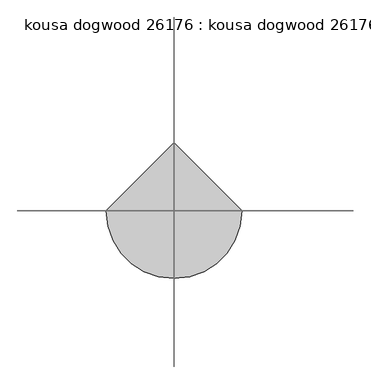
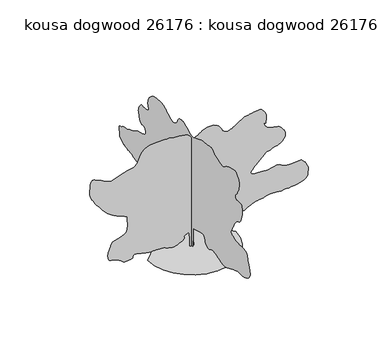
"""IFC4 building model written with IfcOpenShell, lengths in millimetres: proxy geometry, kousa dogwood 26176 : kousa dogwood 26176."""

from ifc_helpers import new_model, si_unit, origin, place, context, project, spatial, triangles, source, transform, mapped, element, save


def kousa_dogwood_26176_kousa_dogwood_26176_6f0fc0eb(model_context):
    return source(origin(), model_context, "Body", "Tessellation", [
        triangles([(0.0326291, 49.3377043, 0.0034665), (0.0326291, -50.8601768, 0.0034665), (0.0326291, -57.1220357, 331.9092828), (0.0326291, -57.1220357, 475.9424606), (0.0326291, -182.3693916, 513.516657), (0.0326291, -389.0262543, 582.4014421), (0.0326291, -489.2241354, 594.9261864), (0.0326291, -501.2738723, 584.1362563), (0.0326291, -513.1610827, 573.0186936), (0.0326291, -524.7180808, 561.2407062), (0.0326291, -535.7823037, 548.4797482), (0.0326291, -546.1886816, 534.4031001), (0.0326291, -555.7746517, 518.6830204), (0.0326291, -564.3725281, 500.9919491), (0.0326291, -570.4532979, 482.6074244), (0.0326291, -573.902615, 465.0966837), (0.0326291, -576.6965941, 448.573964), (0.0326291, -580.8037926, 433.1460176), (0.0326291, -588.2002524, 418.9245747), (0.0326291, -600.8519875, 406.0163146), (0.0326291, -620.7350761, 394.5304241), (0.0326291, -644.1412056, 383.9411722), (0.0326291, -666.1223494, 374.2282113), (0.0326291, -686.7903465, 366.2678687), (0.0326291, -706.251804, 360.9389425), (0.0326291, -724.6185608, 359.1126732), (0.0326291, -742.0023108, 361.6679315), (0.0326291, -758.5046465, 369.4834791), (0.0326291, -775.1569004, 379.6689039), (0.0326291, -792.794632, 388.8713219), (0.0326291, -811.2528076, 397.2532957), (0.0326291, -830.3688646, 404.9748811), (0.0326291, -849.9750807, 412.2062711), (0.0326291, -869.9141253, 419.1074487), (0.0326291, -890.0156599, 425.8435201), (0.0326291, -1008.9993856, 407.0551683), (0.0326291, -1041.2065767, 396.3388893), (0.0326291, -1073.4136951, 385.7318696), (0.0326291, -1105.6183428, 375.3432595), (0.0326291, -1137.8255339, 365.2823184), (0.0326291, -1170.032725, 355.6608127), (0.0326291, -1202.2373726, 346.587929), (0.0326291, -1234.4445637, 338.1703832), (0.0326291, -1267.7464554, 329.9534792), (0.0326291, -1303.0194477, 322.2852336), (0.0326291, -1339.935799, 316.4813364), (0.0326291, -1378.1679131, 313.8524271), (0.0326291, -1417.3854321, 315.7142684), (0.0326291, -1457.2609051, 323.382514), (0.0326291, -1497.4639744, 338.1703832), (0.0326291, -1798.0576904, 463.4177527), (0.0326291, -1820.2750843, 473.4227743), (0.0326291, -1840.0844856, 482.1121422), (0.0326291, -1859.675441, 489.7092802), (0.0326291, -1881.2374969, 496.4275475), (0.0326291, -1906.9626709, 502.488006), (0.0326291, -1939.0428349, 508.1115726), (0.0326291, -1979.6650646, 513.516657), (0.0326291, -2025.1640316, 517.2225354), (0.0326291, -2069.8934235, 518.6271372), (0.0326291, -2113.0912228, 519.2672144), (0.0326291, -2153.987709, 520.6743959), (0.0326291, -2191.8183941, 524.3802381), (0.0326291, -2225.8138481, 531.9189494), (0.0326291, -2255.2066761, 544.8272458), (0.0326291, -2282.9789635, 559.6176584), (0.0326291, -2311.7343304, 572.6529456), (0.0326291, -2340.1594849, 585.2513409), (0.0326291, -2366.9437511, 598.7234837), (0.0326291, -2390.7715118, 614.3901873), (0.0326291, -2410.3243881, 633.559584), (0.0326291, -2424.2918495, 657.5498348), (0.0326291, -2435.5745911, 680.3717703), (0.0326291, -2447.0782494, 697.4989952), (0.0326291, -2457.4845909, 712.4315866), (0.0326291, -2465.4806145, 728.6825569), (0.0326291, -2469.7527374, 749.7518377), (0.0326291, -2468.9856331, 779.1472092), (0.0326291, -2461.8660095, 820.3714371), (0.0326291, -2451.1117241, 863.1297283), (0.0326291, -2440.248143, 897.1276531), (0.0326291, -2429.166116, 925.8652159), (0.0326291, -2417.7564926, 952.8475805), (0.0326291, -2405.9073612, 981.5851433), (0.0326291, -2393.5095715, 1015.5830681), (0.0326291, -2380.4565891, 1058.3413593), (0.0326291, -2369.079958, 1104.2416826), (0.0326291, -2359.2400063, 1144.8817165), (0.0326291, -2347.0987415, 1179.6085213), (0.0326291, -2328.8234035, 1207.76189), (0.0326291, -2300.578616, 1228.6838688), (0.0326291, -2258.5314732, 1241.7191196), (0.0326291, -2198.8465988, 1246.21245), (0.0326291, -2132.0421009, 1246.3038689), (0.0326291, -2070.825634, 1246.94133), (0.0326291, -2014.6459236, 1248.6762531), (0.0326291, -1962.9595436, 1252.05439), (0.0326291, -1915.2150742, 1257.6220734), (0.0326291, -1870.8667637, 1265.9304325), (0.0326291, -1829.3682793, 1277.5230389), (0.0326291, -1789.1296017, 1289.3542934), (0.0326291, -1750.5318123, 1299.3237431), (0.0326291, -1715.9876999, 1309.4000175), (0.0326291, -1687.9080185, 1321.5614845), (0.0326291, -1668.7006153, 1337.7743031), (0.0326291, -1660.7782791, 1360.0120445), (0.0326291, -1666.546677, 1390.2455189), (0.0326291, -1677.3009624, 1417.6496601), (0.0326291, -1684.3291672, 1433.8802101), (0.0326291, -1690.0442253, 1444.6346409), (0.0326291, -1696.8539841, 1455.6073723), (0.0326291, -1707.1689068, 1472.4958763), (0.0326291, -1723.4020729, 1500.9971889), (0.0326291, -1747.9587135, 1546.8060207), (0.0326291, -1772.6957211, 1595.4241287), (0.0326291, -1790.2065708, 1631.3371983), (0.0326291, -1803.9910492, 1658.7057312), (0.0326291, -1817.5547562, 1681.6927002), (0.0326291, -1834.4076519, 1704.4587524), (0.0326291, -1858.0499588, 1731.1693314), (0.0326291, -1891.9919277, 1765.9877003), (0.0326291, -1930.3865318, 1797.7731148), (0.0326291, -1965.2784428, 1817.0720821), (0.0326291, -1996.9903152, 1830.5645725), (0.0326291, -2025.8549778, 1844.9333176), (0.0326291, -2052.2023521, 1866.8611942), (0.0326291, -2076.3577091, 1903.0281727), (0.0326291, -2098.6487904, 1960.119746), (0.0326291, -2116.6878056, 2031.8721977), (0.0326291, -2127.9349388, 2104.7193501), (0.0326291, -2132.4993404, 2174.3915508), (0.0326291, -2130.4901608, 2236.6139156), (0.0326291, -2122.0193115, 2287.1141762), (0.0326291, -2107.193327, 2321.6200642), (0.0326291, -2086.1239735, 2335.8617821), (0.0326291, -2061.2395912, 2337.8150059), (0.0326291, -2035.0395916, 2338.4550831), (0.0326291, -2007.744746, 2337.9979889), (0.0326291, -1979.5736458, 2336.6644947), (0.0326291, -1950.7445915, 2334.6756626), (0.0326291, -1921.4787907, 2332.2473225), (0.0326291, -1891.9919277, 2329.5982109), (0.0326291, -1876.0712425, 2337.7591953), (0.0326291, -1861.2452579, 2346.5781338), (0.0326291, -1848.6112907, 2356.7126896), (0.0326291, -1839.2640415, 2368.8157299), (0.0326291, -1834.2983562, 2383.5502956), (0.0326291, -1834.8089355, 2401.5691086), (0.0326291, -1841.8929508, 2423.534919), (0.0326291, -1852.3552483, 2443.6188675), (0.0326291, -1862.7057793, 2457.6749863), (0.0326291, -1873.6074394, 2468.8865112), (0.0326291, -1885.7104797, 2480.4259232), (0.0326291, -1899.6779411, 2495.4703537), (0.0326291, -1916.1650162, 2517.1948997), (0.0326291, -1935.8271881, 2548.7874481), (0.0326291, -1957.993713, 2590.5450737), (0.0326291, -1979.7208752, 2638.9828148), (0.0326291, -1998.2679989, 2691.5859993), (0.0326291, -2010.9044369, 2745.8149567), (0.0326291, -2014.8847172, 2799.1805946), (0.0326291, -2007.4704895, 2849.1676598), (0.0326291, -1985.926165, 2893.2111923), (0.0326291, -1958.3391861, 2933.0637016), (0.0326291, -1933.1628159, 2970.5032768), (0.0326291, -1908.2047462, 3003.1422729), (0.0326291, -1881.275576, 3028.5424667), (0.0326291, -1850.1809624, 3044.2903427), (0.0326291, -1812.7363003, 3047.9988373), (0.0326291, -1766.7444855, 3037.2547256), (0.0326291, -1719.9146404, 3021.5318481), (0.0326291, -1679.6556152, 3010.4066551), (0.0326291, -1643.3412621, 3001.5929489), (0.0326291, -1608.3425262, 2992.7792427), (0.0326291, -1572.0281731, 2981.6540497), (0.0326291, -1531.7692932, 2965.9314629), (0.0326291, -1484.9393028, 2943.2999954), (0.0326291, -1440.4816967, 2916.7571388), (0.0326291, -1406.1028358, 2891.9665009), (0.0326291, -1377.3093899, 2870.6814629), (0.0326291, -1349.6132607, 2854.6539528), (0.0326291, -1318.5211178, 2845.6370613), (0.0326291, -1279.542247, 2845.383007), (0.0326291, -1228.1834633, 2855.64459), (0.0326291, -1169.5400225, 2873.0182388), (0.0326291, -1113.3069723, 2891.9412117), (0.0326291, -1061.8923054, 2910.8388954), (0.0326291, -1017.7090284, 2928.2378334), (0.0326291, -983.1650614, 2942.5381233), (0.0326291, -960.6707949, 2952.2663086), (0.0326291, -952.6393084, 2955.8221962), (0.0326291, -948.2019339, 2961.3084892), (0.0326291, -935.5502352, 2975.1262505), (0.0326291, -915.6670738, 2993.2870605), (0.0326291, -889.5406889, 3011.93069), (0.0326291, -858.1564127, 3027.043721), (0.0326291, -822.4999409, 3034.7144737), (0.0326291, -783.5541349, 3030.98069), (0.0326291, -732.8176243, 3019.9825241), (0.0326291, -666.742079, 3008.8573311), (0.0326291, -593.7679358, 2998.2911156), (0.0326291, -522.3253853, 2988.9184319), (0.0326291, -460.8523207, 2981.4252846), (0.0326291, -417.7815848, 2976.4215202), (0.0326291, -401.5509622, 2974.6181419), (0.0326291, -395.4346567, 2971.4177559), (0.0326291, -378.6935274, 2962.8581039), (0.0326291, -353.7354941, 2950.4629303), (0.0326291, -322.9710202, 2935.781559), (0.0326291, -288.8105872, 2920.3130264), (0.0326291, -253.665385, 2905.606366), (0.0326291, -219.943588, 2893.2111923), (0.0326291, -185.6193204, 2880.5875443), (0.0326291, -147.7895892, 2865.9061729), (0.0326291, -107.5499033, 2851.6314629), (0.0326291, -65.995522, 2840.3283737), (0.0326291, -24.2222429, 2834.5118683), (0.0326291, 16.6747373, 2836.696328), (0.0326291, 55.5998176, 2849.370845), (0.0326291, 96.5882904, 2870.80849), (0.0326291, 142.7253362, 2895.8528915), (0.0326291, 191.4912912, 2922.0149574), (0.0326291, 240.3669598, 2946.7291466), (0.0326291, 286.8319289, 2967.506076), (0.0326291, 328.3685105, 2981.806366), (0.0326291, 362.4553107, 2987.1403427), (0.0326291, 393.9487736, 2986.9371574), (0.0326291, 428.0736528, 2985.5401497), (0.0326291, 462.85387, 2981.7302078), (0.0326291, 496.3208679, 2974.2879295), (0.0326291, 526.4986044, 2962.0450722), (0.0326291, 551.4210657, 2943.757235), (0.0326291, 569.1121734, 2918.2555939), (0.0326291, 580.8698133, 2890.5442039), (0.0326291, 590.3287926, 2866.0079109), (0.0326291, 599.0181241, 2843.9859993), (0.0326291, 608.4770671, 2823.8439148), (0.0326291, 620.2347433, 2804.8700729), (0.0326291, 635.8252161, 2786.4804977), (0.0326291, 656.7853466, 2767.9638954), (0.0326291, 681.9998686, 2750.4126411), (0.0326291, 708.9670452, 2735.7312698), (0.0326291, 737.1382181, 2724.4281807), (0.0326291, 765.9671997, 2717.0623512), (0.0326291, 794.9054043, 2714.1921776), (0.0326291, 823.4041735, 2716.3766373), (0.0326291, 850.9200085, 2724.1235481), (0.0326291, 879.0352255, 2736.1376404), (0.0326291, 909.4516829, 2750.4632195), (0.0326291, 941.7859011, 2766.6939148), (0.0326291, 975.6542553, 2784.4483543), (0.0326291, 1010.6731934, 2803.3716179), (0.0326291, 1046.4566923, 2823.0564629), (0.0326291, 1082.6262869, 2843.1223892), (0.0326291, 1105.6488642, 2859.0990303), (0.0326291, 1129.9312483, 2874.4405357), (0.0326291, 1156.7333187, 2888.4614822), (0.0326291, 1187.3148823, 2900.5264435), (0.0326291, 1222.9358185, 2909.9244164), (0.0326291, 1264.8559341, 2916.0711342), (0.0326291, 1314.3325653, 2918.2555939), (0.0326291, 1371.27938, 2917.0364822), (0.0326291, 1432.4959923, 2913.0739334), (0.0326291, 1494.5887138, 2905.9365784), (0.0326291, 1554.1644379, 2895.1924667), (0.0326291, 1607.8243893, 2880.384359), (0.0326291, 1652.170229, 2861.0803047), (0.0326291, 1683.8110302, 2836.8486443), (0.0326291, 1706.8716866, 2813.1250923), (0.0326291, 1727.9587715, 2794.2021194), (0.0326291, 1747.4024975, 2778.0222931), (0.0326291, 1765.5329315, 2762.5028915), (0.0326291, 1782.6754898, 2745.5611931), (0.0326291, 1799.1625648, 2725.1141853), (0.0326291, 1815.3220436, 2699.0791466), (0.0326291, 1829.1980862, 2669.9198799), (0.0326291, 1838.9110107, 2641.4210381), (0.0326291, 1844.8978546, 2613.4558846), (0.0326291, 1847.6003059, 2585.9476799), (0.0326291, 1847.4555473, 2558.7696877), (0.0326291, 1844.8978546, 2531.8024384), (0.0326291, 1840.3715321, 2504.9444847), (0.0326291, 1833.1045338, 2480.6264923), (0.0326291, 1823.6481342, 2460.6875931), (0.0326291, 1814.4075645, 2444.1470329), (0.0326291, 1807.7985203, 2430.0144653), (0.0326291, 1806.2288486, 2417.3094269), (0.0326291, 1812.1088676, 2405.0386642), (0.0326291, 1827.8467152, 2392.2218594), (0.0326291, 1849.0074875, 2380.5911739), (0.0326291, 1869.8380474, 2372.0289059), (0.0326291, 1890.7803738, 2365.7678055), (0.0326291, 1912.2687424, 2361.0382977), (0.0326291, 1934.7451321, 2357.0758942), (0.0326291, 1958.643964, 2353.1134907), (0.0326291, 1984.4047462, 2348.386599), (0.0326291, 2010.8612709, 2347.0174965), (0.0326291, 2036.5483658, 2351.2338089), (0.0326291, 2061.4708271, 2357.423838), (0.0326291, 2085.6261841, 2361.9705082), (0.0326291, 2109.0119659, 2361.2567436), (0.0326291, 2131.6332596, 2351.673317), (0.0326291, 2153.4873035, 2329.5982109), (0.0326291, 2174.467709, 2301.4448421), (0.0326291, 2194.0205853, 2275.3743404), (0.0326291, 2211.4933559, 2250.398394), (0.0326291, 2226.2277763, 2225.5318886), (0.0326291, 2237.5638577, 2199.7865124), (0.0326291, 2244.8485874, 2172.181802), (0.0326291, 2247.424157, 2141.7271202), (0.0326291, 2244.3202766, 2107.6962032), (0.0326291, 2235.6283653, 2070.3785683), (0.0326291, 2222.2832497, 2030.3202576), (0.0326291, 2205.211908, 1988.0724003), (0.0326291, 2185.3465508, 1944.1813293), (0.0326291, 2163.6220047, 1899.1954124), (0.0326291, 2140.962632, 1853.6608372), (0.0326291, 2100.9601318, 1858.6798622), (0.0326291, 2062.4918404, 1861.6211071), (0.0326291, 2027.0919662, 1860.3969086), (0.0326291, 1996.2893406, 1852.9291958), (0.0326291, 1971.6234043, 1837.1381538), (0.0326291, 1954.62575, 1810.9380089), (0.0326291, 1946.8304409, 1772.2488007), (0.0326291, 1948.600827, 1732.3757984), (0.0326291, 1958.6973038, 1702.4699203), (0.0326291, 1976.2436165, 1680.2321789), (0.0326291, 2000.3608944, 1663.3615517), (0.0326291, 2030.175499, 1649.5591965), (0.0326291, 2064.8108849, 1636.5213295), (0.0326291, 2103.3883266, 1621.95187), (0.0326291, 2140.6348904, 1609.5186172), (0.0326291, 2173.6091858, 1602.2338875), (0.0326291, 2204.9375061, 1596.8135788), (0.0326291, 2237.2539928, 1589.965741), (0.0326291, 2273.1847939, 1578.4087429), (0.0326291, 2315.3589638, 1558.8558666), (0.0326291, 2366.4078827, 1528.0176327), (0.0326291, 2421.2184906, 1494.715741), (0.0326291, 2472.8516762, 1468.6452393), (0.0326291, 2521.195237, 1447.82994), (0.0326291, 2566.1355171, 1430.3039749), (0.0326291, 2607.5882195, 1414.0911564), (0.0326291, 2645.408876, 1397.2203838), (0.0326291, 2679.5210381, 1377.7208473), (0.0326291, 2712.7951698, 1361.3810017), (0.0326291, 2747.8218109, 1352.8187336), (0.0326291, 2784.0419838, 1348.3076717), (0.0326291, 2820.9228722, 1344.1268223), (0.0326291, 2857.9052078, 1336.5499592), (0.0326291, 2894.4558838, 1321.8536179), (0.0326291, 2930.0159225, 1296.3112816), (0.0326291, 2963.8993195, 1273.2151623), (0.0326291, 2994.8366753, 1263.3725945), (0.0326291, 3021.3795319, 1259.3391197), (0.0326291, 3042.1314629, 1253.6596699), (0.0326291, 3055.6443008, 1238.8896412), (0.0326291, 3060.4954582, 1207.5790524), (0.0326291, 3055.2632195, 1152.2755966), (0.0326291, 3048.7862892, 1092.8295158), (0.0326291, 3047.8970993, 1050.9093275), (0.0326291, 3048.2020226, 1021.8085602), (0.0326291, 3045.3318489, 1000.8104233), (0.0326291, 3034.917659, 983.2107708), (0.0326291, 3012.5405365, 964.2953556), (0.0326291, 2973.8562698, 939.3576336), (0.0326291, 2933.444783, 915.1285892), (0.0326291, 2905.0729683, 899.6650709), (0.0326291, 2883.1527946, 890.2264755), (0.0326291, 2862.1215202, 884.0720547), (0.0326291, 2836.3661156, 878.4662922), (0.0326291, 2800.3488373, 870.6709831), (0.0326291, 2748.4057869, 857.9455971), (0.0326291, 2691.3322357, 845.6215673), (0.0326291, 2642.1070427, 839.1038692), (0.0326291, 2598.7236443, 835.7638115), (0.0326291, 2559.0490311, 832.969796), (0.0326291, 2521.0123993, 828.0955296), (0.0326291, 2482.5441078, 818.5095594), (0.0326291, 2441.5562027, 801.5855925), (0.0326291, 2391.4573711, 781.9767603), (0.0326291, 2330.6243111, 765.8731647), (0.0326291, 2264.4218113, 752.9471369), (0.0326291, 2198.2193115, 742.8683916), (0.0326291, 2137.3862514, 735.3094053), (0.0326291, 2087.2872746, 729.9423637), (0.0326291, 2053.2919659, 726.4371998), (0.0326291, 2029.7944176, 724.3187971), (0.0326291, 2007.1732693, 722.5281361), (0.0326291, 1984.7704216, 719.8636185), (0.0326291, 1961.9308273, 715.1163792), (0.0326291, 1937.993771, 707.0823492), (0.0326291, 1912.3068214, 694.5576777), (0.0326291, 1884.2067924, 676.3382229), (0.0326291, 1858.0626034, 656.8386864), (0.0326291, 1836.8484913, 639.9679865), (0.0326291, 1817.821455, 623.755168), (0.0326291, 1798.2507019, 606.2291665), (0.0326291, 1775.39076, 585.4139036), (0.0326291, 1746.508366, 559.3433292), (0.0326291, 1708.8605186, 526.0414012), (0.0326291, 1676.508569, 493.7427913), (0.0326291, 1660.1509918, 470.1004844), (0.0326291, 1652.0077389, 452.2620747), (0.0326291, 1644.3013779, 437.3827503), (0.0326291, 1629.2594181, 422.612649), (0.0326291, 1599.097015, 405.1019082), (0.0326291, 1546.0389164, 382.0082233), (0.0326291, 1485.3507603, 359.4225743), (0.0326291, 1435.5083084, 343.959056), (0.0326291, 1393.5527298, 333.5323305), (0.0326291, 1356.5270828, 326.0647631), (0.0326291, 1321.4725365, 319.4759937), (0.0326291, 1285.4325851, 311.6781775), (0.0326291, 1245.4478165, 300.5961868), (0.0326291, 1210.2637722, 289.989149), (0.0326291, 1186.3649403, 283.9820483), (0.0326291, 1167.396258, 281.0432742), (0.0326291, 1147.00259, 279.6361108), (0.0326291, 1118.8314171, 278.2314909), (0.0326291, 1076.5277493, 275.2927168), (0.0326291, 1013.7389946, 269.2856162), (0.0326291, 949.454183, 262.3285553), (0.0326291, 902.807103, 257.3450841), (0.0326291, 867.6611378, 254.0024466), (0.0326291, 837.8821415, 251.9765346), (0.0326291, 807.338657, 250.9359004), (0.0326291, 769.8914515, 250.5523664), (0.0326291, 719.4089951, 250.4975006), (0.0326291, 670.7350039, 250.8810346), (0.0326291, 638.2738312, 252.0311461), (0.0326291, 615.2309063, 253.9485981), (0.0326291, 594.8195068, 256.6313377), (0.0326291, 570.2450257, 260.0831982), (0.0326291, 534.7155084, 264.2996015), (0.0326291, 481.4390365, 269.2856162), (0.0326291, 422.1935612, 275.3282706), (0.0326291, 372.4781364, 282.356439), (0.0326291, 331.088875, 289.8240427), (0.0326291, 296.8192008, 297.1824235), (0.0326291, 268.4651902, 303.8829412), (0.0326291, 244.8218659, 309.3794806), (0.0326291, 224.683742, 313.1209311), (0.0326291, 205.1661288, 317.0832982), (0.0326291, 184.3343335, 323.3443986), (0.0326291, 162.4067657, 331.5257306), (0.0326291, 139.6031703, 341.2386915), (0.0326291, 116.1419661, 352.1022726), (0.0326291, 92.2428616, 363.7303782), (0.0326291, 68.1245527, 375.7445795), (0.0326291, 30.5505993, 319.3845386), (45.9178458, 0.0001554, 0.0), (-48.0174088, 0.0001554, 0.0), (-48.0174088, 0.0001413, 231.707096), (-66.8047659, 0.0001319, 375.7420361), (-192.0516131, 0.0001366, 306.8547438), (-187.0307895, 0.0001366, 290.7155763), (-184.0912524, 0.0001413, 274.3554557), (-185.3145244, 0.0001413, 257.5609684), (-192.7818556, 0.0001413, 240.1056022), (-208.5748052, 0.0001413, 221.774926), (-234.7743869, 0.0001413, 202.348768), (-273.4613787, 0.000146, 181.6081554), (-312.0033031, 0.000146, 163.7156429), (-338.7139546, 0.000146, 151.9577214), (-357.1009864, 0.000146, 144.8010271), (-370.6645844, 0.000146, 140.711115), (-382.9175428, 0.000146, 138.1553662), (-397.3574318, 0.000146, 135.5991178), (-417.4970819, 0.000146, 131.5094601), (-439.9710008, 0.000146, 127.9491487), (-460.0369998, 0.000146, 127.5656056), (-479.1149414, 0.000146, 129.7020032), (-498.6322821, 0.000146, 133.7002148), (-520.011464, 0.000146, 138.9039124), (-544.6799074, 0.000146, 144.6549786), (-574.0550039, 0.000146, 150.296313), (-600.4913263, 0.000146, 156.3397305), (-618.3855829, 0.000146, 163.3689162), (-632.2235464, 0.000146, 170.83652), (-646.5008726, 0.000146, 178.1941378), (-665.7083485, 0.000146, 184.8946554), (-694.3366882, 0.000146, 190.3901957), (-736.8765335, 0.000146, 194.1328815), (-779.2336138, 0.000146, 196.4333588), (-808.1184786, 0.000146, 197.9667499), (-829.223295, 0.000146, 198.7340904), (-848.2479332, 0.000146, 198.7335817), (-870.8868856, 0.000146, 197.9670043), (-902.8375517, 0.000146, 196.4333588), (-949.79704, 0.000146, 194.1328815), (-1001.8670448, 0.000146, 193.9319671), (-1046.5989801, 0.000146, 197.8938619), (-1085.8521074, 0.0001413, 204.8138429), (-1121.4908478, 0.0001413, 213.4858971), (-1155.3769335, 0.0001413, 222.706101), (-1189.3723148, 0.0001413, 231.2689323), (-1225.3411949, 0.0001413, 237.9694499), (-1262.0569771, 0.0001413, 244.9072168), (-1296.6897469, 0.0001413, 253.5978201), (-1328.6963688, 0.0001413, 261.9602639), (-1357.5252777, 0.0001413, 267.9114813), (-1382.6281059, 0.0001413, 269.3719663), (-1403.4611366, 0.0001413, 264.2614861), (-1419.473386, 0.0001413, 250.4939398), (-1428.6553837, 0.0001413, 232.4919499), (-1432.3612621, 0.0001413, 216.1330829), (-1435.0815903, 0.0001413, 201.5273247), (-1441.3072277, 0.000146, 188.7833897), (-1455.5312141, 0.000146, 178.0117724), (-1482.2417931, 0.000146, 169.3208967), (-1525.9322948, 0.000146, 162.8212934), (-1572.1602871, 0.000146, 158.3478564), (-1605.9016869, 0.000146, 156.1751329), (-1630.7681923, 0.000146, 157.0702273), (-1650.3770245, 0.000146, 161.7986996), (-1668.3424976, 0.000146, 171.1283627), (-1688.2789261, 0.000146, 185.8258122), (-1713.8033855, 0.0001413, 206.6576257), (-1741.6290127, 0.0001413, 228.2925696), (-1766.9325554, 0.0001413, 245.5460223), (-1791.0319565, 0.0001413, 259.4050238), (-1815.2432693, 0.0001413, 270.8502554), (-1840.8770245, 0.0001366, 280.8756246), (-1869.2486938, 0.0001366, 290.4590512), (-1901.6743309, 0.0001366, 300.5936434), (-1934.6105473, 0.0001366, 309.1178687), (-1963.4954121, 0.0001366, 315.1249875), (-1988.1053925, 0.0001366, 321.4622824), (-2008.2248039, 0.0001366, 330.9745651), (-2023.6349098, 0.0001366, 346.5117345), (-2034.1149387, 0.0001319, 370.9211457), (-2039.4464447, 0.0001319, 407.0526249), (-2041.6181145, 0.0001272, 446.4530906), (-2042.2581917, 0.0001272, 479.9378926), (-2040.5971012, 0.0001272, 509.2596494), (-2035.8675934, 0.0001225, 536.1709428), (-2027.3053253, 0.0001225, 562.4243548), (-2014.1404312, 0.0001225, 589.7750473), (-1995.6085682, 0.0001177, 619.9731314), (-1980.7851997, 0.0001177, 650.0441883), (-1975.1615604, 0.000113, 676.4982422), (-1972.6038677, 0.000113, 700.3234594), (-1966.9802284, 0.000113, 722.5077885), (-1952.15686, 0.000113, 744.0343088), (-1921.9943115, 0.0001083, 765.8884254), (-1870.3612713, 0.0001083, 789.0557613), (-1806.3862518, 0.0001083, 810.6356215), (-1745.0427578, 0.0001083, 829.0404573), (-1688.9546116, 0.0001036, 847.2243038), (-1640.7555187, 0.0001036, 868.148826), (-1603.0720631, 0.0001036, 894.7679861), (-1578.5331539, 9.89e-05, 930.0409784), (-1569.7701714, 9.89e-05, 976.9267794), (-1568.1268124, 9.42e-05, 1021.8771606), (-1564.291436, 9.42e-05, 1052.8067408), (-1559.9098721, 8.95e-05, 1074.8614992), (-1556.6231541, 8.95e-05, 1093.190177), (-1556.0769665, 8.95e-05, 1112.9462385), (-1559.9098721, 8.95e-05, 1139.2733379), (-1569.7701714, 8.48e-05, 1177.3225416), (-1576.8720634, 8.48e-05, 1216.5579374), (-1575.2108276, 8.01e-05, 1245.0591774), (-1570.5906155, 8.01e-05, 1265.8897373), (-1568.8202293, 8.01e-05, 1282.1204327), (-1575.7036755, 8.01e-05, 1296.8193901), (-1597.0446693, 7.54e-05, 1313.0499401), (-1638.6549202, 7.54e-05, 1333.8805), (-1689.8308662, 7.54e-05, 1356.3188107), (-1736.7343987, 7.54e-05, 1376.128212), (-1780.4605087, 7.06e-05, 1394.5153164), (-1822.1063679, 7.06e-05, 1412.6813587), (-1862.7666767, 7.06e-05, 1431.8329514), (-1903.5361359, 7.06e-05, 1453.1765614), (-1945.5097366, 6.59e-05, 1477.916185), (-1986.0430183, 6.59e-05, 1504.27882), (-2022.850074, 6.59e-05, 1530.8625172), (-2057.5770241, 6.12e-05, 1559.4171696), (-2091.8644661, 6.12e-05, 1591.6954319), (-2127.355759, 5.65e-05, 1629.4525749), (-2165.6971687, 5.65e-05, 1674.4409626), (-2208.5291473, 5.18e-05, 1728.408308), (-2247.4724098, 5.18e-05, 1776.3914257), (-2275.4631432, 4.71e-05, 1807.0619373), (-2296.1108654, 4.71e-05, 1827.6587906), (-2313.0348324, 4.71e-05, 1845.4032017), (-2329.849649, 4.24e-05, 1867.5316475), (-2350.1721004, 4.24e-05, 1901.2730473), (-2377.6117046, 3.77e-05, 1953.8535587), (-2407.4999966, 3.77e-05, 2006.0531342), (-2432.6789829, 3.3e-05, 2040.17547), (-2453.0345718, 3.3e-05, 2065.75574), (-2468.4624092, 3.3e-05, 2092.3190895), (-2478.8510193, 2.83e-05, 2129.400547), (-2484.0911064, 2.35e-05, 2186.5275833), (-2484.0733749, 1.88e-05, 2273.2330467), (-2479.4530174, 1.41e-05, 2366.311377), (-2470.8907494, 9.4e-06, 2437.3702663), (-2458.274659, 9.4e-06, 2488.1626602), (-2441.4951599, 4.7e-06, 2520.4409225), (-2420.4462994, 4.7e-06, 2535.9603241), (-2395.0132587, 4.7e-06, 2536.4710487), (-2365.0895039, 4.7e-06, 2523.7276405), (-2332.9179211, 4.7e-06, 2506.6766464), (-2300.967255, 4.7e-06, 2492.3612411), (-2269.456097, 9.4e-06, 2479.6916656), (-2238.6001316, 9.4e-06, 2467.5682777), (-2208.6205662, 9.4e-06, 2454.8963768), (-2179.7381721, 9.4e-06, 2440.583297), (-2152.1690701, 9.4e-06, 2423.5298321), (-2125.5118309, 1.41e-05, 2406.5702568), (-2099.1846588, 1.41e-05, 2392.8949287), (-2073.1318886, 1.41e-05, 2381.9576603), (-2047.2975643, 1.41e-05, 2373.2125546), (-2021.6258755, 1.41e-05, 2366.1106625), (-1996.0658077, 1.41e-05, 2360.1036163), (-1970.5616959, 1.41e-05, 2354.6450832), (-1682.4901806, 9.4e-06, 2454.8428917), (-1632.6478741, 9.4e-06, 2469.2295135), (-1581.2713589, 9.4e-06, 2480.9872261), (-1530.6618027, 4.7e-06, 2491.3200256), (-1483.1180477, 4.7e-06, 2501.43685), (-1440.9440231, 4.7e-06, 2512.5364632), (-1406.4381351, 4.7e-06, 2525.8283844), (-1381.8990807, 4.7e-06, 2542.5137032), (-1363.5324692, 4.7e-06, 2562.071521), (-1346.1512627, 0.0, 2583.1536644), (-1329.9739071, 0.0, 2605.7848412), (-1315.2216099, 0.0, 2629.9403435), (-1302.1126717, -4.7e-06, 2655.6198807), (-1290.8681545, -4.7e-06, 2682.8484512), (-1281.7012722, -4.7e-06, 2711.6013474), (-1272.2067936, -9.4e-06, 2740.658876), (-1260.192556, -9.4e-06, 2768.370266), (-1246.2073631, -9.4e-06, 2794.2529884), (-1230.799728, -1.41e-05, 2817.7224861), (-1214.5132221, -1.41e-05, 2838.2203629), (-1197.8990473, -1.41e-05, 2855.2129303), (-1181.5033911, -1.41e-05, 2868.1667908), (-1163.6852926, -1.41e-05, 2881.2479691), (-1141.7016054, -1.88e-05, 2897.732428), (-1114.4626431, -1.88e-05, 2915.6394745), (-1080.868618, -1.88e-05, 2933.0131233), (-1039.824757, -1.88e-05, 2947.8465202), (-990.2363594, -1.88e-05, 2958.2098412), (-931.0086519, -1.88e-05, 2962.0959412), (-864.0771996, -1.88e-05, 2963.4167908), (-794.2957758, -2.35e-05, 2966.4648605), (-724.9537874, -2.35e-05, 2969.9698792), (-659.3354816, -2.35e-05, 2972.6115784), (-600.7300836, -2.35e-05, 2973.0435287), (-552.4192969, -2.35e-05, 2969.9698792), (-517.694963, -1.88e-05, 2962.0959412), (-488.7008752, -1.88e-05, 2953.1299187), (-455.9831411, -1.88e-05, 2947.1099373), (-420.4180882, -1.88e-05, 2943.1985481), (-382.8794638, -1.88e-05, 2940.4806908), (-344.2460661, -1.88e-05, 2938.0930458), (-305.3942225, -1.88e-05, 2935.146714), (-267.2002783, -1.88e-05, 2930.7777946), (-229.4246408, -1.88e-05, 2925.621714), (-191.9784526, -1.88e-05, 2920.2621574), (-155.9561965, -1.88e-05, 2913.6834892), (-122.4536084, -1.88e-05, 2904.920652), (-92.5659433, -1.88e-05, 2892.9827179), (-67.3887146, -1.41e-05, 2876.8790497), (-48.0174088, -1.41e-05, 2855.64459), (-32.0237993, -1.41e-05, 2832.3274086), (-16.6875397, -1.41e-05, 2811.1185287), (-2.6657036, -9.4e-06, 2792.5257683), (9.3842547, -9.4e-06, 2777.1333939), (18.8051623, -9.4e-06, 2765.4492233), (24.9396909, -9.4e-06, 2758.0325249), (27.1304911, -9.4e-06, 2755.4416946), (33.4842979, -9.4e-06, 2757.6005745), (50.354212, -9.4e-06, 2763.6205559), (74.4544806, -9.4e-06, 2772.6883163), (102.4981041, -9.4e-06, 2784.0675636), (131.1990775, -9.4e-06, 2796.9705551), (157.2708873, -1.41e-05, 2810.6360001), (177.4273059, -1.41e-05, 2824.3264435), (198.7521307, -1.41e-05, 2840.0743195), (228.4025557, -1.41e-05, 2859.1243195), (263.2023211, -1.41e-05, 2879.3681419), (299.971334, -1.88e-05, 2898.7483543), (335.5389304, -1.88e-05, 2915.1569458), (366.7225285, -1.88e-05, 2926.5359024), (390.3470312, -1.88e-05, 2930.7777946), (540.6438529, -1.88e-05, 2924.5293388), (567.3722723, -1.88e-05, 2911.0929497), (593.4453538, -1.88e-05, 2897.5292427), (618.2027452, -1.41e-05, 2883.7623505), (640.986529, -1.41e-05, 2869.6655365), (661.1439468, -1.41e-05, 2855.1367722), (678.0146467, -1.41e-05, 2840.0490303), (690.9406746, -1.41e-05, 2824.3264435), (701.3114805, -1.41e-05, 2808.0451698), (711.0244778, -9.4e-06, 2791.4333931), (720.188744, -9.4e-06, 2774.5425636), (728.9161909, -9.4e-06, 2757.4229691), (737.3134254, -9.4e-06, 2740.1507675), (745.4947575, -4.7e-06, 2722.7774094), (753.564323, -4.7e-06, 2705.3276024), (770.998942, -4.7e-06, 2693.3387993), (788.3801485, -4.7e-06, 2681.8325249), (805.652132, -4.7e-06, 2671.3168877), (822.7590094, -4.7e-06, 2662.2744164), (839.6474407, -4.7e-06, 2655.2132195), (856.2616156, -4.7e-06, 2650.6158257), (872.5480488, 0.0, 2648.9650543), (890.1477013, -4.7e-06, 2650.5143784), (910.5972525, -4.7e-06, 2655.1117722), (933.675713, -4.7e-06, 2662.7825249), (959.1620207, -4.7e-06, 2673.5013474), (986.8404184, -4.7e-06, 2687.3188179), (1016.4923876, -4.7e-06, 2704.1846489), (1047.8943953, -4.7e-06, 2724.1235481), (1083.8810795, -9.4e-06, 2748.583683), (1125.6716972, -9.4e-06, 2777.209552), (1170.63981, -1.41e-05, 2807.2577179), (1216.1565811, -1.41e-05, 2836.0103233), (1259.5905579, -1.41e-05, 2860.6992233), (1298.3153744, -1.41e-05, 2878.5809807), (1329.6996506, -1.88e-05, 2886.9374474), (1357.4515903, -1.88e-05, 2890.1887024), (1386.8470345, -1.88e-05, 2894.4050148), (1417.611581, -1.88e-05, 2899.434359), (1449.4706829, -1.88e-05, 2905.1238373), (1482.1503742, -1.88e-05, 2911.3214241), (1515.3785786, -1.88e-05, 2917.8239342), (1548.8838009, -1.88e-05, 2924.5293388), (1579.6278545, -1.88e-05, 2928.4157295), (1609.6633759, -1.88e-05, 2931.4635086), (1638.271368, -1.88e-05, 2932.9113853), (1664.7457695, -1.88e-05, 2931.8701698), (1688.3703449, -1.88e-05, 2927.5265396), (1708.4362713, -1.88e-05, 2919.0939148), (1724.2274586, -1.88e-05, 2905.7333931), (1739.6377098, -1.88e-05, 2887.4455559), (1757.7860207, -1.41e-05, 2865.1951698), (1776.8105862, -1.41e-05, 2839.6679489), (1794.8496014, -1.41e-05, 2811.5248993), (1810.0387905, -9.4e-06, 2781.4005753), (1820.5188194, -9.4e-06, 2749.9554016), (1824.4254124, -4.7e-06, 2717.8498032), (1823.8792248, -4.7e-06, 2687.1156326), (1822.3451614, -4.7e-06, 2658.9978722), (1819.9880379, 0.0, 2633.0645714), (1816.9755764, 0.0, 2608.9090691), (1813.4704124, 0.0, 2586.0491272), (1809.6375069, 4.7e-06, 2564.0527954), (1805.6394951, 4.7e-06, 2542.5137032), (1792.4214066, 4.7e-06, 2547.6189148), (1780.407169, 4.7e-06, 2551.2003822), (1770.80354, 4.7e-06, 2551.7084908), (1764.8142254, 4.7e-06, 2547.6189148), (1763.6456921, 4.7e-06, 2537.4029686), (1768.502227, 4.7e-06, 2519.5113281), (1780.590152, 4.7e-06, 2492.4170517), (1797.6232693, 9.4e-06, 2463.2045906), (1815.644553, 9.4e-06, 2439.6894562), (1833.3357697, 9.4e-06, 2421.4318497), (1849.383482, 1.41e-05, 2407.9926991), (1862.4745434, 1.41e-05, 2398.9375832), (1871.2934818, 1.41e-05, 2393.8245232), (1874.5243893, 1.41e-05, 2392.2192432), (2006.0352573, 1.41e-05, 2360.9061836), (2106.2332111, 1.41e-05, 2342.1204117), (2156.332188, 1.88e-05, 2317.0709232), (2184.3204506, 1.88e-05, 2284.955151), (2211.1580566, 2.35e-05, 2253.3880371), (2235.6969658, 2.35e-05, 2222.9156239), (2256.7840508, 2.35e-05, 2194.0867149), (2273.2711258, 2.83e-05, 2167.449678), (2284.005209, 2.83e-05, 2143.5508461), (2287.8405853, 2.83e-05, 2122.9387321), (2287.548452, 2.83e-05, 2101.2852573), (2285.5038094, 3.3e-05, 2074.7017056), (2279.9538574, 3.3e-05, 2044.3943985), (2269.1462322, 3.77e-05, 2011.5674778), (2251.3255177, 3.77e-05, 1977.4247944), (2224.7419659, 3.77e-05, 1943.1728153), (2187.6427769, 4.24e-05, 1910.0182983), (2148.5165314, 4.24e-05, 1884.4557598), (2115.4153542, 4.24e-05, 1869.632246), (2085.9284912, 4.24e-05, 1861.707439), (2057.6480953, 4.71e-05, 1856.8510494), (2028.1612324, 4.71e-05, 1851.2274101), (1995.0625259, 4.71e-05, 1841.0039062), (1955.9364258, 4.71e-05, 1822.3451614), (1919.2562519, 4.71e-05, 1805.0172947), (1892.545673, 4.71e-05, 1797.98909), (1871.969022, 4.71e-05, 1796.2187038), (1853.6938293, 4.71e-05, 1794.6667637), (1833.8842827, 4.71e-05, 1788.2938969), (1808.7052963, 5.18e-05, 1772.0633469), (1774.3264355, 5.18e-05, 1740.9331249), (1505.0459244, 6.59e-05, 1484.1772854), (1485.271986, 7.06e-05, 1456.1332123), (1467.6368706, 7.06e-05, 1428.9120541), (1454.2714073, 7.06e-05, 1403.3342548), (1447.31689, 7.54e-05, 1380.2176426), (1448.9042931, 7.54e-05, 1360.3903645), (1461.1725849, 7.54e-05, 1344.6703938), (1486.2601524, 7.54e-05, 1333.8805), (1518.9396984, 7.54e-05, 1327.8936562), (1552.9350071, 7.54e-05, 1325.0819092), (1588.7947369, 7.54e-05, 1324.0226715), (1627.0624592, 7.54e-05, 1323.2911755), (1668.2865417, 7.54e-05, 1321.4649788), (1713.0185497, 7.54e-05, 1317.1214939), (1761.8017639, 7.54e-05, 1308.8310116), (1817.2701805, 7.54e-05, 1306.5500462), (1879.6373039, 7.54e-05, 1316.6465229), (1945.839949, 7.54e-05, 1332.3285599), (2012.806937, 7.54e-05, 1346.8064552), (2077.4753735, 7.54e-05, 1353.2886177), (2136.7766956, 7.54e-05, 1344.9827293), (2187.6427769, 7.54e-05, 1315.0945827), (2246.979562, 8.01e-05, 1283.7104519), (2327.2410873, 8.01e-05, 1271.0561371), (2418.6734425, 8.01e-05, 1270.5634346), (2511.5307106, 8.01e-05, 1275.6586178), (2596.0566559, 8.01e-05, 1279.7657799), (2662.5284706, 8.01e-05, 1276.3139557), (2701.1618683, 8.01e-05, 1258.7320347), (2721.1516365, 8.01e-05, 1235.3818611), (2738.3982582, 8.48e-05, 1217.6171024), (2753.2319458, 8.48e-05, 1203.3575077), (2766.0082008, 8.48e-05, 1190.5228987), (2777.0063667, 8.48e-05, 1177.030481), (2786.6075249, 8.48e-05, 1160.7998583), (2795.0910187, 8.95e-05, 1139.7483089), (2804.082621, 8.95e-05, 1118.5139219), (2814.1918877, 8.95e-05, 1101.005761), (2824.1741272, 8.95e-05, 1084.0436422), (2832.8355171, 9.42e-05, 1064.4526142), (2839.0075241, 9.42e-05, 1039.0577253), (2841.4207489, 9.42e-05, 1004.6787918), (2838.931366, 9.89e-05, 958.1409348), (2835.7565598, 0.0001036, 909.1367311), (2833.5973892, 0.0001036, 868.2402449), (2827.2727753, 0.0001036, 833.5870548), (2811.6010574, 0.0001083, 803.3152834), (2781.5020226, 0.0001083, 775.563271), (2731.7943008, 0.000113, 748.4691399), (2657.321521, 0.000113, 720.1710125), (2574.4414055, 0.000113, 695.9978514), (2501.0708839, 0.000113, 680.9178125), (2434.5027088, 0.0001177, 672.5181072), (2371.9906815, 0.0001177, 668.393141), (2310.7894753, 0.0001177, 666.1274363), (2248.1658268, 0.0001177, 663.3156893), (2181.3790604, 0.0001177, 657.5472914), (2119.1770432, 0.0001177, 654.5704382), (2068.6945141, 0.0001177, 659.0433483), (2024.7830956, 0.0001177, 666.9122721), (1982.2990608, 0.000113, 674.1258579), (1936.0888, 0.000113, 676.6252693), (1881.0064064, 0.0001177, 670.3641689), (1811.9005955, 0.0001177, 651.2836475), (1743.30798, 0.0001177, 630.3794729), (1690.270229, 0.0001177, 619.0053852), (1648.4034531, 0.0001177, 613.6561478), (1613.3311752, 0.0001177, 610.8265966), (1580.6693607, 0.0001177, 607.0089518), (1546.0338295, 0.0001177, 598.7031724), (1505.0459244, 0.0001225, 582.3988987), (1466.4506058, 0.0001225, 564.4157304), (1439.3564747, 0.0001225, 552.017977), (1419.9280094, 0.0001225, 543.1279673), (1404.3375366, 0.0001225, 535.6603998), (1388.7444477, 0.0001225, 527.5349147), (1369.3185986, 0.0001225, 516.6713699), (1342.2243221, 0.0001272, 500.9894056), (1315.7879997, 0.0001272, 485.3607811), (1297.8963593, 0.0001272, 474.8807522), (1284.0557796, 0.0001272, 467.7967006), (1269.7784534, 0.0001272, 462.356008), (1250.5710503, 0.0001272, 456.8061287), (1221.9427105, 0.0001272, 449.3918647), (1179.4027925, 0.0001272, 438.3657208), (910.1222815, 0.0001319, 388.2667803), (853.5971706, 0.0001319, 374.6828711), (809.1217604, 0.0001319, 365.4804531), (771.108165, 0.0001319, 359.6740125), (733.9733677, 0.0001366, 356.2780352), (692.1268667, 0.0001366, 354.3070072), (639.9832472, 0.0001366, 352.7728349), (571.9544417, 0.0001366, 350.6925839), (496.5875668, 0.0001366, 348.7367804), (426.8087228, 0.0001366, 348.0992466), (363.600844, 0.0001366, 348.5564498), (307.9494807, 0.0001366, 349.8874005), (260.8451975, 0.0001366, 351.8787761), (223.271746, 0.0001366, 354.3070072), (196.2139136, 0.0001366, 356.9536843), (175.2909174, 0.0001319, 361.2818358), (155.3537078, 0.0001319, 368.5665656), (136.2379233, 0.0001319, 378.3150621), (117.7795024, 0.0001319, 390.0371664), (99.8140837, 0.0001319, 403.2375235), (82.177097, 0.0001319, 417.4234308), (64.7046942, 0.0001319, 432.102077), (39.6552239, 0.0001272, 513.5116064), (27.1304911, 0.0001366, 294.3299995), (-1074.6684877, 0.0, 0.0031651), (-1046.2560505, -246.2427458, 0.0031651), (-965.3444195, -472.3763266, 0.0031651), (-838.405438, -671.9262829, 0.0031651), (-671.9262829, -838.4079088, 0.0031651), (-472.3763266, -965.3444195, 0.0031651), (-246.2427458, -1046.2560505, 0.0031651), (4.7e-05, -1074.6684877, 0.0031651), (246.2430001, -1046.2560505, 0.0031651), (472.3763266, -965.3444195, 0.0031651), (671.9262829, -838.405438, 0.0031651), (838.4079088, -671.9262829, 0.0031651), (965.3444195, -472.3763266, 0.0031651), (1046.2560505, -246.2427458, 0.0031651), (1074.6684877, 9.42e-05, 0.0031651), (-0.0001409, 1074.6684877, 0.0031651)], [[451, 1, 2], [451, 2, 3], [451, 3, 4], [450, 451, 4], [316, 317, 318], [316, 318, 319], [315, 316, 319], [356, 357, 358], [355, 356, 358], [354, 355, 358], [354, 358, 359], [353, 354, 359], [353, 359, 360], [133, 134, 135], [133, 135, 136], [132, 133, 136], [132, 136, 137], [132, 137, 138], [131, 132, 138], [131, 138, 139], [131, 139, 140], [130, 131, 140], [130, 140, 141], [130, 141, 142], [129, 130, 142], [128, 129, 142], [127, 128, 142], [126, 127, 142], [125, 126, 142], [124, 125, 142], [123, 124, 142], [122, 123, 142], [122, 142, 143], [121, 122, 143], [121, 143, 144], [121, 144, 145], [120, 121, 145], [119, 120, 145], [119, 145, 146], [118, 119, 146], [315, 319, 320], [314, 315, 320], [313, 314, 320], [312, 313, 320], [311, 312, 320], [310, 311, 320], [309, 310, 320], [308, 309, 320], [307, 308, 320], [306, 307, 320], [305, 306, 320], [304, 305, 320], [304, 320, 321], [303, 304, 321], [302, 303, 321], [301, 302, 321], [300, 301, 321], [299, 300, 321], [298, 299, 321], [297, 298, 321], [296, 297, 321], [295, 296, 321], [294, 295, 321], [293, 294, 321], [292, 293, 321], [292, 321, 322], [291, 292, 322], [290, 291, 322], [289, 290, 322], [289, 322, 323], [288, 289, 323], [352, 353, 360], [352, 360, 361], [117, 118, 146], [351, 352, 361], [350, 351, 361], [349, 350, 361], [348, 349, 361], [347, 348, 361], [347, 361, 362], [347, 362, 363], [347, 363, 364], [347, 364, 365], [347, 365, 366], [347, 366, 367], [347, 367, 368], [347, 368, 369], [347, 369, 370], [347, 370, 371], [347, 371, 372], [347, 372, 373], [347, 373, 374], [346, 347, 374], [346, 374, 375], [346, 375, 376], [345, 346, 376], [345, 376, 377], [344, 345, 377], [343, 344, 377], [343, 377, 378], [342, 343, 378], [341, 342, 378], [341, 378, 379], [340, 341, 379], [340, 379, 380], [340, 380, 381], [339, 340, 381], [339, 381, 382], [339, 382, 383], [338, 339, 383], [338, 383, 384], [337, 338, 384], [337, 384, 385], [336, 337, 385], [335, 336, 385], [334, 335, 385], [333, 334, 385], [333, 385, 386], [332, 333, 386], [332, 386, 387], [332, 387, 388], [331, 332, 388], [331, 388, 389], [331, 389, 390], [330, 331, 390], [329, 330, 390], [329, 390, 391], [328, 329, 391], [328, 391, 392], [328, 392, 393], [327, 328, 393], [327, 393, 394], [327, 394, 395], [327, 395, 396], [326, 327, 396], [326, 396, 397], [326, 397, 398], [326, 398, 399], [326, 399, 400], [326, 400, 401], [326, 401, 402], [325, 326, 402], [288, 323, 324], [116, 117, 146], [116, 146, 147], [115, 116, 147], [114, 115, 147], [113, 114, 147], [112, 113, 147], [111, 112, 147], [110, 111, 147], [325, 402, 403], [204, 205, 206], [167, 168, 169], [167, 169, 170], [166, 167, 170], [165, 166, 170], [165, 170, 171], [164, 165, 171], [164, 171, 172], [163, 164, 172], [162, 163, 172], [161, 162, 172], [160, 161, 172], [159, 160, 172], [158, 159, 172], [158, 172, 173], [157, 158, 173], [157, 173, 174], [156, 157, 174], [156, 174, 175], [155, 156, 175], [155, 175, 176], [154, 155, 176], [153, 154, 176], [152, 153, 176], [152, 176, 177], [151, 152, 177], [151, 177, 178], [151, 178, 179], [150, 151, 179], [150, 179, 180], [149, 150, 180], [149, 180, 181], [148, 149, 181], [148, 181, 182], [147, 148, 182], [110, 147, 182], [110, 182, 183], [110, 183, 184], [110, 184, 185], [110, 185, 186], [109, 110, 186], [109, 186, 187], [108, 109, 187], [108, 187, 188], [107, 108, 188], [107, 188, 189], [107, 189, 190], [107, 190, 191], [106, 107, 191], [89, 90, 91], [89, 91, 92], [88, 89, 92], [88, 92, 93], [87, 88, 93], [87, 93, 94], [86, 87, 94], [86, 94, 95], [85, 86, 95], [84, 85, 95], [84, 95, 96], [83, 84, 96], [83, 96, 97], [82, 83, 97], [81, 82, 97], [80, 81, 97], [79, 80, 97], [78, 79, 97], [77, 78, 97], [76, 77, 97], [75, 76, 97], [74, 75, 97], [73, 74, 97], [72, 73, 97], [71, 72, 97], [70, 71, 97], [69, 70, 97], [68, 69, 97], [67, 68, 97], [66, 67, 97], [65, 66, 97], [64, 65, 97], [63, 64, 97], [62, 63, 97], [61, 62, 97], [60, 61, 97], [59, 60, 97], [58, 59, 97], [57, 58, 97], [57, 97, 98], [56, 57, 98], [56, 98, 99], [55, 56, 99], [55, 99, 100], [54, 55, 100], [54, 100, 101], [53, 54, 101], [53, 101, 102], [52, 53, 102], [51, 52, 102], [50, 51, 102], [50, 102, 103], [50, 103, 104], [50, 104, 105], [49, 50, 105], [48, 49, 105], [47, 48, 105], [46, 47, 105], [45, 46, 105], [44, 45, 105], [43, 44, 105], [42, 43, 105], [41, 42, 105], [40, 41, 105], [39, 40, 105], [38, 39, 105], [37, 38, 105], [36, 37, 105], [35, 36, 105], [35, 105, 106], [35, 106, 191], [34, 35, 191], [33, 34, 191], [32, 33, 191], [31, 32, 191], [30, 31, 191], [29, 30, 191], [28, 29, 191], [27, 28, 191], [26, 27, 191], [25, 26, 191], [24, 25, 191], [23, 24, 191], [22, 23, 191], [21, 22, 191], [20, 21, 191], [19, 20, 191], [18, 19, 191], [17, 18, 191], [16, 17, 191], [15, 16, 191], [14, 15, 191], [13, 14, 191], [12, 13, 191], [11, 12, 191], [10, 11, 191], [9, 10, 191], [8, 9, 191], [7, 8, 191], [6, 7, 191], [5, 6, 191], [5, 191, 192], [5, 192, 193], [5, 193, 194], [5, 194, 195], [5, 195, 196], [5, 196, 197], [5, 197, 198], [5, 198, 199], [5, 199, 200], [5, 200, 201], [5, 201, 202], [5, 202, 203], [5, 203, 204], [5, 204, 206], [5, 206, 207], [5, 207, 208], [5, 208, 209], [5, 209, 210], [5, 210, 211], [5, 211, 212], [5, 212, 213], [5, 213, 214], [5, 214, 215], [5, 215, 216], [5, 216, 217], [5, 217, 218], [4, 5, 218], [4, 218, 219], [4, 219, 220], [4, 220, 221], [4, 221, 222], [4, 222, 223], [4, 223, 224], [4, 224, 225], [4, 225, 226], [4, 226, 227], [4, 227, 228], [4, 228, 229], [4, 229, 230], [4, 230, 231], [4, 231, 232], [4, 232, 233], [4, 233, 234], [4, 234, 235], [4, 235, 236], [4, 236, 237], [4, 237, 238], [4, 238, 239], [4, 239, 240], [4, 240, 241], [4, 241, 242], [4, 242, 243], [4, 243, 244], [4, 244, 245], [450, 4, 245], [449, 450, 245], [448, 449, 245], [447, 448, 245], [446, 447, 245], [445, 446, 245], [444, 445, 245], [443, 444, 245], [442, 443, 245], [441, 442, 245], [440, 441, 245], [439, 440, 245], [438, 439, 245], [437, 438, 245], [436, 437, 245], [435, 436, 245], [434, 435, 245], [433, 434, 245], [432, 433, 245], [431, 432, 245], [430, 431, 245], [429, 430, 245], [428, 429, 245], [427, 428, 245], [426, 427, 245], [425, 426, 245], [424, 425, 245], [423, 424, 245], [422, 423, 245], [422, 245, 246], [421, 422, 246], [420, 421, 246], [419, 420, 246], [418, 419, 246], [417, 418, 246], [416, 417, 246], [415, 416, 246], [414, 415, 246], [413, 414, 246], [412, 413, 246], [411, 412, 246], [410, 411, 246], [409, 410, 246], [408, 409, 246], [407, 408, 246], [406, 407, 246], [405, 406, 246], [404, 405, 246], [403, 404, 246], [325, 403, 246], [324, 325, 246], [288, 324, 246], [288, 246, 247], [288, 247, 248], [288, 248, 249], [287, 288, 249], [287, 249, 250], [287, 250, 251], [287, 251, 252], [287, 252, 253], [287, 253, 254], [287, 254, 255], [287, 255, 256], [287, 256, 257], [287, 257, 258], [287, 258, 259], [287, 259, 260], [287, 260, 261], [287, 261, 262], [287, 262, 263], [286, 287, 263], [286, 263, 264], [286, 264, 265], [286, 265, 266], [286, 266, 267], [286, 267, 268], [286, 268, 269], [286, 269, 270], [285, 286, 270], [285, 270, 271], [285, 271, 272], [285, 272, 273], [285, 273, 274], [285, 274, 275], [285, 275, 276], [285, 276, 277], [285, 277, 278], [285, 278, 279], [285, 279, 280], [285, 280, 281], [285, 281, 282], [284, 285, 282], [284, 282, 283], [751, 752, 753], [906, 452, 453], [906, 453, 454], [906, 454, 455], [905, 906, 455], [751, 753, 754], [750, 751, 754], [750, 754, 755], [749, 750, 755], [600, 601, 602], [599, 600, 602], [599, 602, 603], [598, 599, 603], [598, 603, 604], [597, 598, 604], [597, 604, 605], [597, 605, 606], [596, 597, 606], [596, 606, 607], [596, 607, 608], [596, 608, 609], [595, 596, 609], [595, 609, 610], [595, 610, 611], [594, 595, 611], [593, 594, 611], [592, 593, 611], [591, 592, 611], [591, 611, 612], [590, 591, 612], [590, 612, 613], [589, 590, 613], [589, 613, 614], [589, 614, 615], [588, 589, 615], [588, 615, 616], [587, 588, 616], [586, 587, 616], [585, 586, 616], [584, 585, 616], [584, 616, 617], [583, 584, 617], [582, 583, 617], [581, 582, 617], [580, 581, 617], [580, 617, 618], [579, 580, 618], [578, 579, 618], [577, 578, 618], [576, 577, 618], [575, 576, 618], [574, 575, 618], [573, 574, 618], [572, 573, 618], [571, 572, 618], [570, 571, 618], [570, 618, 619], [569, 570, 619], [569, 619, 620], [569, 620, 621], [568, 569, 621], [568, 621, 622], [567, 568, 622], [567, 622, 623], [567, 623, 624], [566, 567, 624], [566, 624, 625], [566, 625, 626], [565, 566, 626], [903, 904, 905], [748, 749, 755], [565, 626, 627], [902, 903, 905], [508, 509, 510], [508, 510, 511], [507, 508, 511], [507, 511, 512], [506, 507, 512], [506, 512, 513], [505, 506, 513], [505, 513, 514], [505, 514, 515], [505, 515, 516], [505, 516, 517], [505, 517, 518], [505, 518, 519], [505, 519, 520], [505, 520, 521], [504, 505, 521], [504, 521, 522], [504, 522, 523], [747, 748, 755], [747, 755, 756], [565, 627, 628], [901, 902, 905], [900, 901, 905], [899, 900, 905], [898, 899, 905], [897, 898, 905], [896, 897, 905], [895, 896, 905], [894, 895, 905], [893, 894, 905], [892, 893, 905], [825, 826, 827], [824, 825, 827], [824, 827, 828], [823, 824, 828], [823, 828, 829], [823, 829, 830], [823, 830, 831], [823, 831, 832], [823, 832, 833], [823, 833, 834], [823, 834, 835], [822, 823, 835], [822, 835, 836], [822, 836, 837], [822, 837, 838], [822, 838, 839], [822, 839, 840], [822, 840, 841], [822, 841, 842], [822, 842, 843], [822, 843, 844], [822, 844, 845], [822, 845, 846], [822, 846, 847], [822, 847, 848], [822, 848, 849], [822, 849, 850], [821, 822, 850], [821, 850, 851], [821, 851, 852], [821, 852, 853], [820, 821, 853], [820, 853, 854], [820, 854, 855], [820, 855, 856], [820, 856, 857], [819, 820, 857], [819, 857, 858], [818, 819, 858], [817, 818, 858], [816, 817, 858], [815, 816, 858], [814, 815, 858], [814, 858, 859], [813, 814, 859], [813, 859, 860], [812, 813, 860], [812, 860, 861], [812, 861, 862], [811, 812, 862], [810, 811, 862], [810, 862, 863], [809, 810, 863], [809, 863, 864], [808, 809, 864], [808, 864, 865], [807, 808, 865], [807, 865, 866], [806, 807, 866], [806, 866, 867], [805, 806, 867], [805, 867, 868], [805, 868, 869], [804, 805, 869], [804, 869, 870], [804, 870, 871], [804, 871, 872], [804, 872, 873], [804, 873, 874], [804, 874, 875], [804, 875, 876], [804, 876, 877], [804, 877, 878], [804, 878, 879], [804, 879, 880], [804, 880, 881], [804, 881, 882], [804, 882, 883], [803, 804, 883], [803, 883, 884], [803, 884, 885], [803, 885, 886], [803, 886, 887], [803, 887, 888], [803, 888, 889], [803, 889, 890], [803, 890, 891], [802, 803, 891], [802, 891, 892], [802, 892, 905], [801, 802, 905], [800, 801, 905], [799, 800, 905], [688, 689, 690], [746, 747, 756], [905, 455, 456], [768, 769, 770], [767, 768, 770], [767, 770, 771], [767, 771, 772], [767, 772, 773], [767, 773, 774], [767, 774, 775], [767, 775, 776], [767, 776, 777], [767, 777, 778], [767, 778, 779], [767, 779, 780], [767, 780, 781], [767, 781, 782], [767, 782, 783], [767, 783, 784], [767, 784, 785], [767, 785, 786], [767, 786, 787], [767, 787, 788], [767, 788, 789], [766, 767, 789], [766, 789, 790], [766, 790, 791], [766, 791, 792], [766, 792, 793], [766, 793, 794], [766, 794, 795], [765, 766, 795], [764, 765, 795], [763, 764, 795], [763, 795, 796], [762, 763, 796], [761, 762, 796], [761, 796, 797], [761, 797, 798], [760, 761, 798], [759, 760, 798], [758, 759, 798], [757, 758, 798], [745, 746, 756], [744, 745, 756], [743, 744, 756], [742, 743, 756], [741, 742, 756], [740, 741, 756], [739, 740, 756], [738, 739, 756], [737, 738, 756], [736, 737, 756], [735, 736, 756], [734, 735, 756], [733, 734, 756], [732, 733, 756], [731, 732, 756], [730, 731, 756], [729, 730, 756], [728, 729, 756], [727, 728, 756], [726, 727, 756], [726, 756, 757], [726, 757, 798], [725, 726, 798], [724, 725, 798], [723, 724, 798], [722, 723, 798], [721, 722, 798], [720, 721, 798], [719, 720, 798], [718, 719, 798], [717, 718, 798], [716, 717, 798], [715, 716, 798], [714, 715, 798], [713, 714, 798], [712, 713, 798], [711, 712, 798], [710, 711, 798], [710, 798, 799], [710, 799, 905], [709, 710, 905], [708, 709, 905], [707, 708, 905], [706, 707, 905], [705, 706, 905], [704, 705, 905], [703, 704, 905], [702, 703, 905], [701, 702, 905], [700, 701, 905], [699, 700, 905], [698, 699, 905], [697, 698, 905], [696, 697, 905], [695, 696, 905], [694, 695, 905], [693, 694, 905], [692, 693, 905], [691, 692, 905], [690, 691, 905], [688, 690, 905], [687, 688, 905], [686, 687, 905], [685, 686, 905], [684, 685, 905], [683, 684, 905], [682, 683, 905], [681, 682, 905], [680, 681, 905], [679, 680, 905], [678, 679, 905], [677, 678, 905], [676, 677, 905], [675, 676, 905], [674, 675, 905], [674, 905, 456], [673, 674, 456], [672, 673, 456], [671, 672, 456], [670, 671, 456], [669, 670, 456], [668, 669, 456], [667, 668, 456], [666, 667, 456], [665, 666, 456], [664, 665, 456], [663, 664, 456], [662, 663, 456], [661, 662, 456], [660, 661, 456], [659, 660, 456], [658, 659, 456], [657, 658, 456], [656, 657, 456], [655, 656, 456], [654, 655, 456], [653, 654, 456], [652, 653, 456], [651, 652, 456], [650, 651, 456], [649, 650, 456], [648, 649, 456], [647, 648, 456], [646, 647, 456], [645, 646, 456], [644, 645, 456], [643, 644, 456], [642, 643, 456], [641, 642, 456], [640, 641, 456], [639, 640, 456], [638, 639, 456], [637, 638, 456], [636, 637, 456], [635, 636, 456], [634, 635, 456], [633, 634, 456], [632, 633, 456], [631, 632, 456], [630, 631, 456], [629, 630, 456], [628, 629, 456], [565, 628, 456], [564, 565, 456], [563, 564, 456], [562, 563, 456], [561, 562, 456], [560, 561, 456], [559, 560, 456], [558, 559, 456], [557, 558, 456], [556, 557, 456], [555, 556, 456], [554, 555, 456], [553, 554, 456], [552, 553, 456], [551, 552, 456], [551, 456, 457], [551, 457, 458], [551, 458, 459], [551, 459, 460], [551, 460, 461], [551, 461, 462], [551, 462, 463], [551, 463, 464], [551, 464, 465], [551, 465, 466], [551, 466, 467], [551, 467, 468], [551, 468, 469], [551, 469, 470], [551, 470, 471], [551, 471, 472], [551, 472, 473], [551, 473, 474], [551, 474, 475], [551, 475, 476], [551, 476, 477], [551, 477, 478], [551, 478, 479], [551, 479, 480], [551, 480, 481], [551, 481, 482], [551, 482, 483], [551, 483, 484], [551, 484, 485], [551, 485, 486], [551, 486, 487], [551, 487, 488], [551, 488, 489], [551, 489, 490], [551, 490, 491], [551, 491, 492], [551, 492, 493], [551, 493, 494], [551, 494, 495], [551, 495, 496], [551, 496, 497], [551, 497, 498], [551, 498, 499], [551, 499, 500], [551, 500, 501], [551, 501, 502], [551, 502, 503], [551, 503, 504], [551, 504, 523], [550, 551, 523], [549, 550, 523], [548, 549, 523], [548, 523, 524], [547, 548, 524], [547, 524, 525], [546, 547, 525], [545, 546, 525], [544, 545, 525], [543, 544, 525], [542, 543, 525], [541, 542, 525], [540, 541, 525], [540, 525, 526], [539, 540, 526], [538, 539, 526], [537, 538, 526], [536, 537, 526], [535, 536, 526], [534, 535, 526], [534, 526, 527], [533, 534, 527], [533, 527, 528], [532, 533, 528], [532, 528, 529], [531, 532, 529], [531, 529, 530], [921, 922, 907], [920, 921, 907], [920, 907, 908], [919, 920, 908], [919, 908, 909], [919, 909, 910], [918, 919, 910], [917, 918, 910], [917, 910, 911], [917, 911, 912], [917, 912, 913], [917, 913, 914], [917, 914, 915], [917, 915, 916]], closed=False),
    ])


if __name__ == "__main__":
    model = new_model("IFC4")
    model_context = context("Model", 3, world=origin())
    ifc_project = project(units=[si_unit("LENGTHUNIT", "METRE", prefix="MILLI")], contexts=[model_context])
    site = spatial("IfcSite", under=ifc_project)
    building = spatial("IfcBuilding", under=site)
    placement = place(None, origin())
    kousa_dogwood_26176_kousa_dogwood_26176_shape = kousa_dogwood_26176_kousa_dogwood_26176_6f0fc0eb(model_context)
    element("IfcBuildingElementProxy", 1, Name="kousa dogwood 26176 : kousa dogwood 26176", ObjectType="kousa dogwood 26176 : kousa dogwood 26176", at=placement, inside=building, context=model_context, shape_type="MappedRepresentation", body=[
        mapped(kousa_dogwood_26176_kousa_dogwood_26176_shape, transform((0.0, 0.0, 0.0), x_axis=(1.0, 0.0, 0.0), y_axis=(0.0, 1.0, 0.0), z_axis=(0.0, 0.0, 1.0))),
    ])
    save(model, "model.ifc")

# Revit data of these elements
# Type "kousa dogwood 26176 : kousa dogwood 26176"
#   built-in parameter 1005195 = "RPC-16-G2M3-G0FX-C7PN-N000-ST1L-LVER-AU"
#   Height = 0
